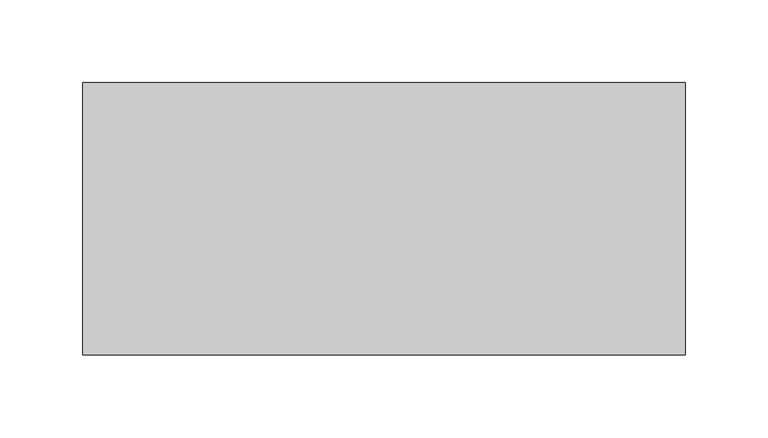
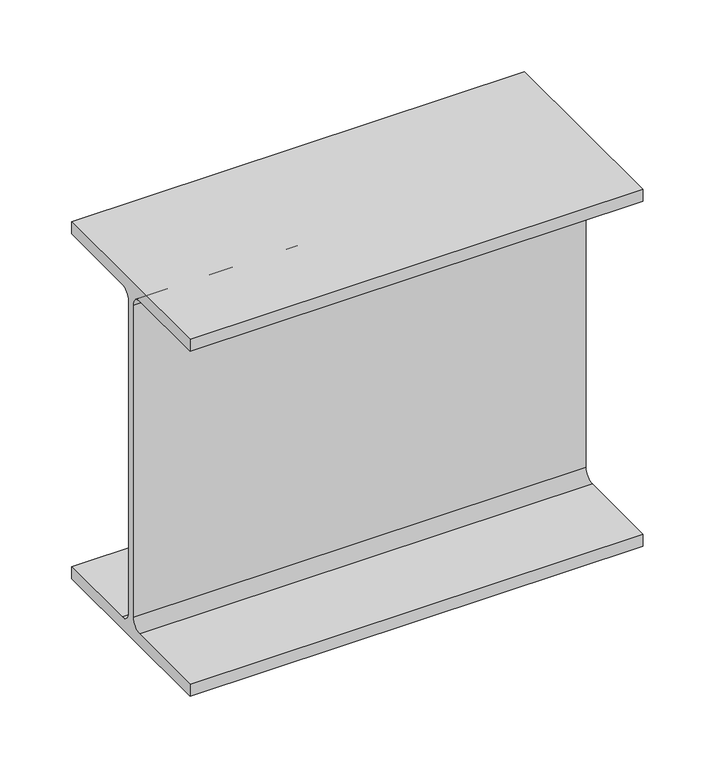
"""IFC4 building model written with IfcOpenShell, lengths in millimetres: beam geometry, Old_Steel Beam_H-KSD3502 : H_SB_ASB_H-300×150x6.5x9."""

import ifcopenshell
import ifcopenshell.guid

model = None  # the IFC model being written
_history = None  # IfcOwnerHistory: only IFC2X3 demands one
_inside = {}  # id of a spatial element -> (the spatial element, [elements in it])
_under = {}  # id of a project, library or spatial element -> (it, [spatial elements below it])
_declared = {}  # id of a project -> (the project, [libraries it declares])
_typed = {}  # id of a type object -> (the type object, [elements of that type])
_made_of = {}  # id of a material, layer set ... -> (it, [elements and type objects made of it])


def new_model(schema):
    """Start an empty IFC model of exactly this schema.

    Asked for "IFC4X3", IfcOpenShell would pick the latest addendum, in which some entities
    have other attributes; the version numbers below select the first issue.
    IFC2X3 requires an IfcOwnerHistory on every rooted entity: one is made here for all.
    """
    global model, _history
    if schema == "IFC4X3":
        model = ifcopenshell.file(schema_version=(4, 3, 0, 0))
    else:
        model = ifcopenshell.file(schema=schema)
    _inside.clear()
    _under.clear()
    _declared.clear()
    _typed.clear()
    _made_of.clear()
    _history = None
    if model.schema == "IFC2X3":
        org = make("IfcOrganization", Name="unknown")
        user = make(
            "IfcPersonAndOrganization",
            ThePerson=make("IfcPerson", FamilyName="unknown"),
            TheOrganization=org,
        )
        app = make(
            "IfcApplication",
            ApplicationDeveloper=org,
            Version="unknown",
            ApplicationFullName="unknown",
            ApplicationIdentifier="unknown",
        )
        _history = make(
            "IfcOwnerHistory",
            OwningUser=user,
            OwningApplication=app,
            ChangeAction="ADDED",
            CreationDate=0,
        )
    return model


def make(cls, **values):
    """One entity of the class cls with the attributes given. An attribute that is None is left unset."""
    return model.create_entity(
        cls, **{name: value for name, value in values.items() if value is not None}
    )


def rooted(cls, **values):
    """An entity with a GlobalId (a new one), such as an element, a storey or a relation."""
    return make(cls, GlobalId=ifcopenshell.guid.new(), OwnerHistory=_history, **values)


def si_unit(unit_type, name, prefix=None):
    """IfcSIUnit, for example si_unit("LENGTHUNIT", "METRE", prefix="MILLI")."""
    return make("IfcSIUnit", UnitType=unit_type, Prefix=prefix, Name=name)


def assignment(units):
    """IfcUnitAssignment: the units of a project."""
    return None if units is None else make("IfcUnitAssignment", Units=units)


def point(xyz):
    """IfcCartesianPoint."""
    return None if xyz is None else make("IfcCartesianPoint", Coordinates=xyz)


def direction(xyz):
    """IfcDirection."""
    return None if xyz is None else make("IfcDirection", DirectionRatios=xyz)


def frame(location, z_axis=None, x_axis=None):
    """IfcAxis2Placement3D, a coordinate frame: its origin and axes. An axis left out is left unset."""
    return make(
        "IfcAxis2Placement3D",
        Location=point(location),
        Axis=direction(z_axis),
        RefDirection=direction(x_axis),
    )


def frame_2d(location, x_axis=None):
    """IfcAxis2Placement2D, a coordinate frame in the plane: its origin and x axis."""
    return make(
        "IfcAxis2Placement2D", Location=point(location), RefDirection=direction(x_axis)
    )


def origin():
    """The frame at (0, 0, 0) with its axes left unset."""
    return frame((0.0, 0.0, 0.0))


def place(relative_to, where):
    """IfcLocalPlacement: puts the frame where relative to a parent placement (None: the world)."""
    return make(
        "IfcLocalPlacement", PlacementRelTo=relative_to, RelativePlacement=where
    )


def context(
    kind, dimensions, precision=None, world=None, true_north=None, identifier=None
):
    """IfcGeometricRepresentationContext, for example the 3D "Model" context."""
    return make(
        "IfcGeometricRepresentationContext",
        ContextIdentifier=identifier,
        ContextType=kind,
        CoordinateSpaceDimension=dimensions,
        Precision=precision,
        WorldCoordinateSystem=world,
        TrueNorth=true_north,
    )


def project(units=None, contexts=None):
    """IfcProject with its units and contexts."""
    return rooted(
        "IfcProject",
        Name="project",
        RepresentationContexts=contexts,
        UnitsInContext=assignment(units),
    )


def spatial(cls, under=None, at=None, **own):
    """A site, building, storey or space (cls), placed at a placement, below another one or the project."""
    s = rooted(cls, ObjectPlacement=at, **own)
    if under is not None:
        _under.setdefault(under.id(), (under, []))[1].append(s)
    return s


def polyline(points):
    """IfcPolyline through the points."""
    return make("IfcPolyline", Points=[point(p) for p in points])


def circle_curve(where, radius):
    """IfcCircle in the frame where."""
    return make("IfcCircle", Position=where, Radius=radius)


def trimmed(basis, trim1, trim2, sense, master):
    """IfcTrimmedCurve: the piece of a basis curve between two trims."""
    return make(
        "IfcTrimmedCurve",
        BasisCurve=basis,
        Trim1=trim1,
        Trim2=trim2,
        SenseAgreement=sense,
        MasterRepresentation=master,
    )


def segment(curve, same_sense, transition):
    """IfcCompositeCurveSegment."""
    return make(
        "IfcCompositeCurveSegment",
        Transition=transition,
        SameSense=same_sense,
        ParentCurve=curve,
    )


def composite_curve(segments, self_intersect=None):
    """IfcCompositeCurve: segments joined end to end."""
    return make("IfcCompositeCurve", Segments=segments, SelfIntersect=self_intersect)


def outline(outer, holes=None, kind="AREA"):
    """IfcArbitraryClosedProfileDef: a profile drawn as a closed curve; with holes, ...WithVoids."""
    if holes is None:
        return make("IfcArbitraryClosedProfileDef", ProfileType=kind, OuterCurve=outer)
    return make(
        "IfcArbitraryProfileDefWithVoids",
        ProfileType=kind,
        OuterCurve=outer,
        InnerCurves=holes,
    )


def extrude(swept, where, along, depth):
    """IfcExtrudedAreaSolid: the profile swept, set in the frame where, extruded along a direction by depth."""
    return make(
        "IfcExtrudedAreaSolid",
        SweptArea=swept,
        Position=where,
        ExtrudedDirection=direction(along),
        Depth=depth,
    )


def shape(context_of_items, identifier, shape_type, items):
    """IfcShapeRepresentation: the items that make up one representation, for example the "Body"."""
    return make(
        "IfcShapeRepresentation",
        ContextOfItems=context_of_items,
        RepresentationIdentifier=identifier,
        RepresentationType=shape_type,
        Items=items,
    )


def source(mapping_origin, context_of_items, identifier, shape_type, items):
    """IfcRepresentationMap: a shape defined once, which mapped items show again and again."""
    return make(
        "IfcRepresentationMap",
        MappingOrigin=mapping_origin,
        MappedRepresentation=shape(context_of_items, identifier, shape_type, items),
    )


def transform(
    local_origin,
    x_axis=None,
    y_axis=None,
    z_axis=None,
    scale=None,
    scale2=None,
    scale3=None,
    uniform=True,
):
    """IfcCartesianTransformationOperator3D, or its non-uniform kind. x_axis, y_axis, z_axis: its Axis1, 2, 3."""
    if uniform:
        return make(
            "IfcCartesianTransformationOperator3D",
            Axis1=direction(x_axis),
            Axis2=direction(y_axis),
            LocalOrigin=point(local_origin),
            Scale=scale,
            Axis3=direction(z_axis),
        )
    return make(
        "IfcCartesianTransformationOperator3DnonUniform",
        Axis1=direction(x_axis),
        Axis2=direction(y_axis),
        LocalOrigin=point(local_origin),
        Scale=scale,
        Axis3=direction(z_axis),
        Scale2=scale2,
        Scale3=scale3,
    )


def mapped(mapping_source, mapping_target):
    """IfcMappedItem: shows the shape of a source again, moved by a transform."""
    return make(
        "IfcMappedItem", MappingSource=mapping_source, MappingTarget=mapping_target
    )


def made_of(thing, what):
    """Note that an element or type object is made of a material, layer set ...; save() writes the relation."""
    if what is not None:
        _made_of.setdefault(what.id(), (what, []))[1].append(thing)
    return thing


def element(
    cls,
    number,
    at=None,
    inside=None,
    cuts=None,
    type_object=None,
    material=None,
    context=None,
    identifier="Body",
    shape_type=None,
    held_by="IfcProductDefinitionShape",
    body=None,
    shapes=None,
    **own,
):
    """One element of the class cls, such as IfcWall. Its Tag is "e" and its number.

    at: its placement. inside: the storey or other place that contains it. cuts: it is an
    opening in that element (IfcRelVoidsElement). A single representation is given by context,
    identifier, shape_type and body (its items); several are given by shapes. held_by: the class
    of the entity that holds the representations. save() writes the other relations.
    """
    e = rooted(cls, Tag="e%d" % number, ObjectPlacement=at, **own)
    if body is not None:
        shapes = [shape(context, identifier, shape_type, body)]
    if shapes is not None:
        e.Representation = make(held_by, Representations=shapes)
    if inside is not None:
        _inside.setdefault(inside.id(), (inside, []))[1].append(e)
    if cuts is not None:
        rooted(
            "IfcRelVoidsElement", RelatingBuildingElement=cuts, RelatedOpeningElement=e
        )
    if type_object is not None:
        _typed.setdefault(type_object.id(), (type_object, []))[1].append(e)
    return made_of(e, material)


def aggregate(whole, parts):
    """IfcRelAggregates: a whole, such as a stair, and the parts it consists of."""
    return rooted("IfcRelAggregates", RelatingObject=whole, RelatedObjects=parts)


def save(model, path):
    """Write the relations noted so far, then the file.

    IfcRelAggregates (storeys below a building ...), IfcRelContainedInSpatialStructure (elements
    in a storey), IfcRelDefinesByType, IfcRelAssociatesMaterial and IfcRelDeclares: one each for
    every whole, place, type object, material and project.
    """
    for whole, parts in _under.values():
        aggregate(whole, parts)
    for where, things in _inside.values():
        rooted(
            "IfcRelContainedInSpatialStructure",
            RelatedElements=things,
            RelatingStructure=where,
        )
    for kind, things in _typed.values():
        rooted("IfcRelDefinesByType", RelatedObjects=things, RelatingType=kind)
    for what, things in _made_of.values():
        rooted("IfcRelAssociatesMaterial", RelatedObjects=things, RelatingMaterial=what)
    for by, libraries in _declared.values():
        rooted("IfcRelDeclares", RelatingContext=by, RelatedDefinitions=libraries)
    model.write(path)


def beam_067efcca(model_context):
    return source(origin(), model_context, "Body", "SweptSolid", [
        extrude(outline(composite_curve([segment(polyline([(82.5, -141.5), (82.5, -151.7), (-82.5, -151.7), (-82.5, -141.5), (-11.9, -141.5)]), True, "CONTINUOUS"), segment(trimmed(circle_curve(frame_2d((-11.9, -132.6)), 8.9), [point((-11.9, -141.5))], [point((-3.0, -132.6))], True, "CARTESIAN"), True, "CONTINUOUS"), segment(polyline([(-3.0, -132.6), (-3.0, 132.6)]), True, "CONTINUOUS"), segment(trimmed(circle_curve(frame_2d((-11.9, 132.6)), 8.9), [point((-3.0, 132.6))], [point((-11.9, 141.5))], True, "CARTESIAN"), True, "CONTINUOUS"), segment(polyline([(-11.9, 141.5), (-82.5, 141.5), (-82.5, 151.7), (82.5, 151.7), (82.5, 141.5), (11.9, 141.5)]), True, "CONTINUOUS"), segment(trimmed(circle_curve(frame_2d((11.9, 132.6)), 8.9), [point((11.9, 141.5))], [point((3.0, 132.6))], True, "CARTESIAN"), True, "CONTINUOUS"), segment(polyline([(3.0, 132.6), (3.0, -132.6)]), True, "CONTINUOUS"), segment(trimmed(circle_curve(frame_2d((11.9, -132.6)), 8.9), [point((3.0, -132.6))], [point((11.9, -141.5))], True, "CARTESIAN"), True, "CONTINUOUS"), segment(polyline([(11.9, -141.5), (82.5, -141.5)]), True, "CONTINUOUS")], self_intersect=False)), frame((-282.3, 0.0, 0.0), z_axis=(1.0, 0.0, 0.0), x_axis=(0.0, 1.0, 0.0)), (0.0, 0.0, 1.0), 364.6),
    ])


if __name__ == "__main__":
    model = new_model("IFC4")
    model_context = context("Model", 3, world=origin())
    ifc_project = project(units=[si_unit("LENGTHUNIT", "METRE", prefix="MILLI")], contexts=[model_context])
    site = spatial("IfcSite", under=ifc_project)
    building = spatial("IfcBuilding", under=site)
    placement = place(None, origin())
    beam_shape = beam_067efcca(model_context)
    element("IfcBeam", 1, ObjectType="Old_Steel Beam_H-KSD3502 : H_SB_ASB_H-300×150x6.5x9", at=placement, inside=building, context=model_context, shape_type="MappedRepresentation", body=[
        mapped(beam_shape, transform((0.0, 0.0, 0.0), x_axis=(1.0, 0.0, 0.0), y_axis=(0.0, 1.0, 0.0), z_axis=(0.0, 0.0, 1.0))),
    ])
    save(model, "model.ifc")

# Revit data of these elements
# Type "Old_Steel Beam_H-KSD3502 : H_SB_ASB_H-300×150x6.5x9"
#   Width = 15.0 cm
#   Web Thickness = 0.65 cm
#   Web Fillet = 1.3 cm
#   Warping Constant = 107174.0 cm⁶
#   Torsional Moment of Inertia = 9.9539 cm⁴
#   Torsional Modulus = 1.0 cm³
#   Section Area = 46.78 cm²
#   Plastic Modulus weak axis = 105.0 cm³
#   Plastic Modulus strong axis = 542.0 cm³
#   Perimeter = 1.17 m²/m
#   Nominal Weight = 36.70 kgf/m
#   Moment of Inertia weak axis = 508.00 cm⁴
#   Moment of Inertia strong axis = 7210.00 cm⁴
#   Height = 30.0 cm
#   Flange Thickness = 0.9 cm
#   Elastic Modulus weak axis = 67.7 cm³
#   Elastic Modulus strong axis = 481.0 cm³
#   Centroid Vertical = 15.0 cm
#   Centroid Horizontal = 7.5 cm
#   Length [instance default] = 1.5240 m
#   Structural Material [instance default] = Steel, 45-345
#   Assembly Code = ""
# Element 1 (IfcBeam, "Old_Steel Beam_H-KSD3502 : H_SB_ASB_H-300×150x6.5x9")
#   Structural Material = none
# Materials
#   "Steel, 45-345": class "Metal", colour RGB 189 187 185, transparency 0, Description = "Steel 345 MPa", Cost = 0
